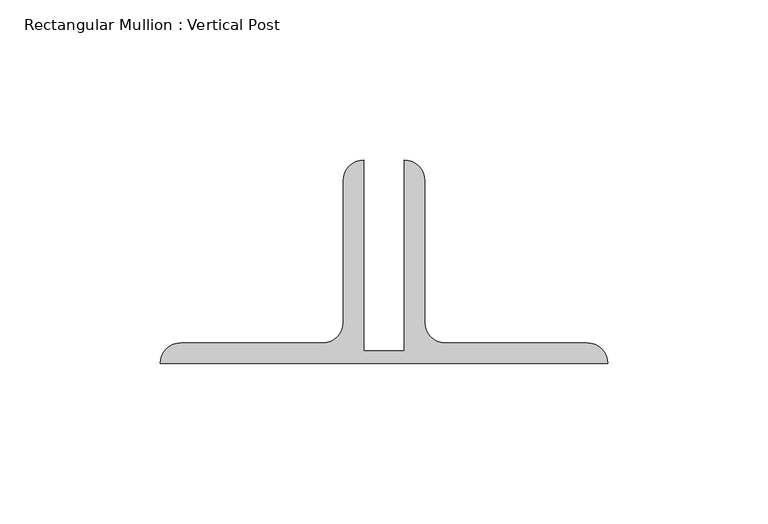
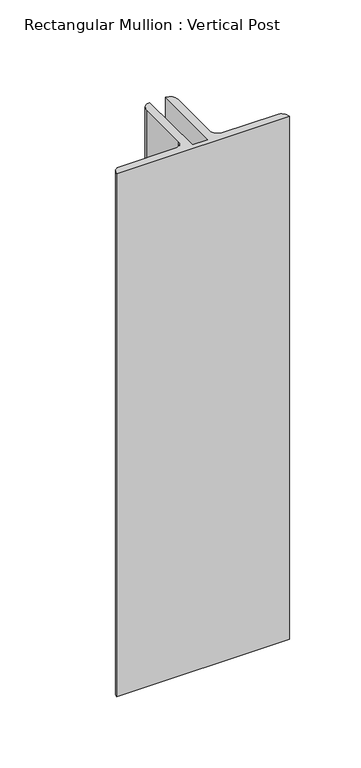
"""IFC4 building model written with IfcOpenShell, lengths in millimetres: member geometry, Rectangular Mullion : Vertical Post."""

from ifc_helpers import new_model, si_unit, point, frame, frame_2d, origin, place, context, project, spatial, polyline, circle_curve, trimmed, segment, composite_curve, outline, extrude, source, transform, mapped, element, save


def rectangular_mullion_vertical_post_d9231392(model_context):
    return source(origin(), model_context, "Body", "SweptSolid", [
        extrude(outline(composite_curve([segment(polyline([(-63.5, 22.9145205), (-63.5, 82.55)]), True, "CONTINUOUS"), segment(trimmed(circle_curve(frame_2d((-63.5, 76.2)), 6.35), [point((-63.5, 82.55))], [point((-57.15, 76.2))], False, "CARTESIAN"), True, "CONTINUOUS"), segment(polyline([(-57.15, 76.2), (-57.15, 31.75)]), True, "CONTINUOUS"), segment(trimmed(circle_curve(frame_2d((-50.8, 31.75)), 6.35), [point((-57.15, 31.75))], [point((-50.8, 25.4))], True, "CARTESIAN"), True, "CONTINUOUS"), segment(polyline([(-50.8, 25.4), (-6.35, 25.4)]), True, "CONTINUOUS"), segment(trimmed(circle_curve(frame_2d((-6.35, 19.05)), 6.35), [point((-6.35, 25.4))], [point((0.0, 19.05))], False, "CARTESIAN"), True, "CONTINUOUS"), segment(polyline([(0.0, 19.05), (-139.7, 19.05)]), True, "CONTINUOUS"), segment(trimmed(circle_curve(frame_2d((-133.35, 19.05)), 6.35), [point((-139.7, 19.05))], [point((-133.35, 25.4))], False, "CARTESIAN"), True, "CONTINUOUS"), segment(polyline([(-133.35, 25.4), (-88.9, 25.4)]), True, "CONTINUOUS"), segment(trimmed(circle_curve(frame_2d((-88.9, 31.75)), 6.35), [point((-88.9, 25.4))], [point((-82.55, 31.75))], True, "CARTESIAN"), True, "CONTINUOUS"), segment(polyline([(-82.55, 31.75), (-82.55, 76.2)]), True, "CONTINUOUS"), segment(trimmed(circle_curve(frame_2d((-76.2, 76.2)), 6.35), [point((-82.55, 76.2))], [point((-76.2, 82.55))], False, "CARTESIAN"), True, "CONTINUOUS"), segment(polyline([(-76.2, 82.55), (-76.2, 22.9145205), (-63.5, 22.9145205)]), True, "CONTINUOUS")], self_intersect=False)), frame((0.0, 0.0, -446.7663052), z_axis=(0.0, 0.0, 1.0), x_axis=(1.0, 0.0, 0.0)), (0.0, 0.0, 1.0), 446.7663052),
    ])


if __name__ == "__main__":
    model = new_model("IFC4")
    model_context = context("Model", 3, world=origin())
    ifc_project = project(units=[si_unit("LENGTHUNIT", "METRE", prefix="MILLI")], contexts=[model_context])
    site = spatial("IfcSite", under=ifc_project)
    building = spatial("IfcBuilding", under=site)
    placement = place(None, origin())
    rectangular_mullion_vertical_post_shape = rectangular_mullion_vertical_post_d9231392(model_context)
    element("IfcMember", 1, ObjectType="Rectangular Mullion : Vertical Post", at=placement, inside=building, context=model_context, shape_type="MappedRepresentation", body=[
        mapped(rectangular_mullion_vertical_post_shape, transform((0.0, 0.0, 0.0), x_axis=(1.0, 0.0, 0.0), y_axis=(0.0, 1.0, 0.0), z_axis=(0.0, 0.0, 1.0))),
    ])
    save(model, "model.ifc")

# Revit data of these elements
# Type "Rectangular Mullion : Vertical Post"
#   built-in parameter 1007351 = -0.0625 (stored number, unit not read)
#   built-in parameter 1007322 = 0.0126789 (stored number, unit not read)
#   built-in parameter 1007321 = 0.229167 (stored number, unit not read)
#   built-in parameter 1007320 = 0.229167 (stored number, unit not read)
# Element 1 (IfcMember, "Rectangular Mullion : Vertical Post")
#   Materials on its faces: "GATE POST: (2) BACK/BACK GALVANIZED ANGLES"
# Materials
#   "GATE POST: (2) BACK/BACK GALVANIZED ANGLES": class "Unassigned", colour RGB 211 211 211, transparency 0, Cost = 0
